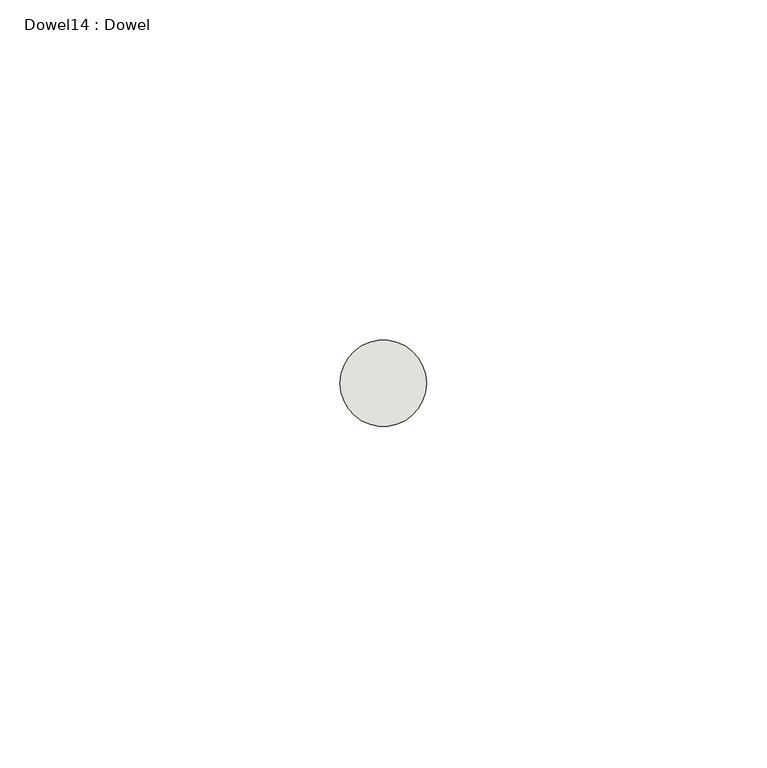
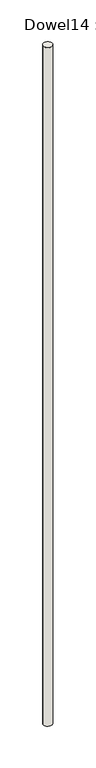
"""IFC4 building model written with IfcOpenShell, lengths in millimetres: wall geometry, Dowel14 : Dowel."""

from ifc_helpers import new_model, si_unit, point, frame, frame_2d, origin, place, context, project, spatial, circle_curve, trimmed, segment, composite_curve, outline, extrude, source, transform, mapped, element, save


def dowel14_dowel_a71a8b82(model_context):
    return source(origin(), model_context, "Body", "SweptSolid", [
        extrude(outline(composite_curve([segment(trimmed(circle_curve(frame_2d((375060.8910859, 446.88125)), 6.35), [point((375054.5410859, 446.88125))], [point((375067.2410859, 446.88125))], False, "CARTESIAN"), True, "CONTINUOUS"), segment(trimmed(circle_curve(frame_2d((375060.8910859, 446.88125)), 6.35), [point((375067.2410859, 446.88125))], [point((375054.5410859, 446.88125))], False, "CARTESIAN"), True, "CONTINUOUS")], self_intersect=False)), frame((0.0, 0.0, 1473.3420731), z_axis=(0.0, 0.0, 1.0), x_axis=(1.0, 0.0, 0.0)), (0.0, 0.0, 1.0), 1016.0),
    ])


if __name__ == "__main__":
    model = new_model("IFC4")
    model_context = context("Model", 3, world=origin())
    ifc_project = project(units=[si_unit("LENGTHUNIT", "METRE", prefix="MILLI")], contexts=[model_context])
    site = spatial("IfcSite", under=ifc_project)
    building = spatial("IfcBuilding", under=site)
    placement = place(None, origin())
    dowel14_dowel_shape = dowel14_dowel_a71a8b82(model_context)
    element("IfcWall", 1, ObjectType="Dowel14 : Dowel", at=placement, inside=building, context=model_context, shape_type="MappedRepresentation", body=[
        mapped(dowel14_dowel_shape, transform((0.0, 0.0, 0.0), x_axis=(1.0, 0.0, 0.0), y_axis=(0.0, 1.0, 0.0), z_axis=(0.0, 0.0, 1.0))),
    ])
    save(model, "model.ifc")

# Revit data of these elements
# Element 1 (IfcWall, "Dowel14 : Dowel")
#   Materials on its faces: "#4 REBARS @ 24\" O.C."
# Materials
#   "#4 REBARS @ 24\" O.C.": class "Generic", colour RGB 255 255 255, transparency 0, Cost = 0
